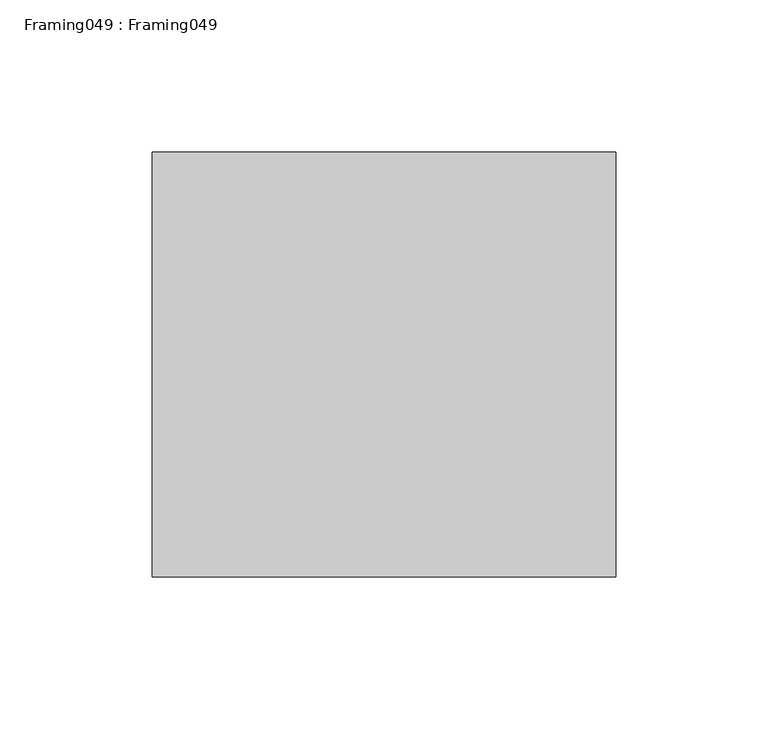
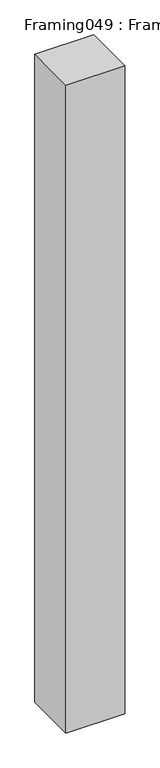
"""IFC4 building model written with IfcOpenShell, lengths in millimetres: proxy geometry, Framing049 : Framing049."""

from ifc_helpers import new_model, si_unit, frame, origin, place, context, project, spatial, polyline, outline, extrude, source, transform, mapped, element, save


def framing049_framing049_c84e7dd9(model_context):
    return source(origin(), model_context, "Body", "SweptSolid", [
        extrude(outline(polyline([(13383.0178845, -4637.5417972), (13383.0178845, -4497.8425368), (13535.4178845, -4497.8425368), (13535.4178845, -4637.5417972), (13383.0178845, -4637.5417972)])), frame((0.0, 0.0, 36582.096), z_axis=(0.0, 0.0, 1.0), x_axis=(1.0, 0.0, 0.0)), (0.0, 0.0, 1.0), 1778.0),
    ])


if __name__ == "__main__":
    model = new_model("IFC4")
    model_context = context("Model", 3, world=origin())
    ifc_project = project(units=[si_unit("LENGTHUNIT", "METRE", prefix="MILLI")], contexts=[model_context])
    site = spatial("IfcSite", under=ifc_project)
    building = spatial("IfcBuilding", under=site)
    placement = place(None, origin())
    framing049_framing049_shape = framing049_framing049_c84e7dd9(model_context)
    element("IfcBuildingElementProxy", 1, Name="Framing049 : Framing049", ObjectType="Framing049 : Framing049", at=placement, inside=building, context=model_context, shape_type="MappedRepresentation", body=[
        mapped(framing049_framing049_shape, transform((0.0, 0.0, 0.0), x_axis=(1.0, 0.0, 0.0), y_axis=(0.0, 1.0, 0.0), z_axis=(0.0, 0.0, 1.0))),
    ])
    save(model, "model.ifc")

# Revit data of these elements
# Type "Framing049 : Framing049"
#   NameOverride = "Framing049"
# Element 1 (IfcBuildingElementProxy, "Framing049 : Framing049")
#   Materials on its faces: "WOOD FRAMING (SEE STRUCT DWGS)"
# Materials
#   "WOOD FRAMING (SEE STRUCT DWGS)": class "Unassigned", colour RGB 224 188 168, transparency 0, Cost = 0
